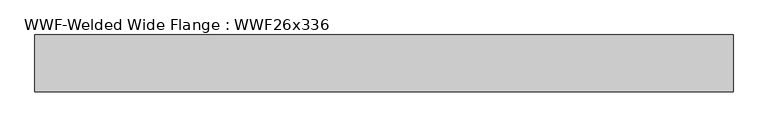
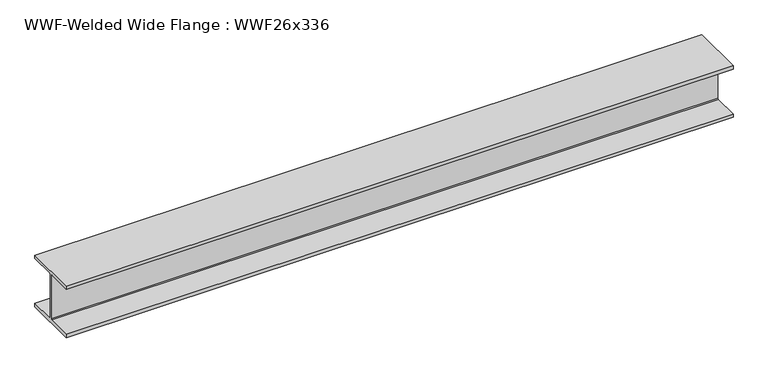
"""IFC4 building model written with IfcOpenShell, lengths in millimetres: beam geometry, WWF-Welded Wide Flange : WWF26x336."""

from ifc_helpers import new_model, si_unit, frame, origin, place, context, project, spatial, polyline, outline, extrude, source, transform, mapped, element, save


def wwf_welded_wide_flange_wwf26x336_1f70f701(model_context):
    return source(origin(), model_context, "Body", "SweptSolid", [
        extrude(outline(polyline([(324.993, -284.988), (324.993, -324.993), (-324.993, -324.993), (-324.993, -284.988), (-20.6375, -284.988), (-9.9949, -274.3454), (-9.9949, 274.3454), (-20.6375, 284.988), (-324.993, 284.988), (-324.993, 324.993), (324.993, 324.993), (324.993, 284.988), (20.6375, 284.988), (9.9949, 274.3454), (9.9949, -274.3454), (20.6375, -284.988), (324.993, -284.988)])), frame((-3934.8877112, 0.0, 0.0), z_axis=(1.0, 0.0, 0.0), x_axis=(0.0, 1.0, 0.0)), (0.0, 0.0, 1.0), 7999.1222788),
    ])


if __name__ == "__main__":
    model = new_model("IFC4")
    model_context = context("Model", 3, world=origin())
    ifc_project = project(units=[si_unit("LENGTHUNIT", "METRE", prefix="MILLI")], contexts=[model_context])
    site = spatial("IfcSite", under=ifc_project)
    building = spatial("IfcBuilding", under=site)
    placement = place(None, origin())
    wwf_welded_wide_flange_wwf26x336_shape = wwf_welded_wide_flange_wwf26x336_1f70f701(model_context)
    element("IfcBeam", 1, ObjectType="WWF-Welded Wide Flange : WWF26x336", at=placement, inside=building, context=model_context, shape_type="MappedRepresentation", body=[
        mapped(wwf_welded_wide_flange_wwf26x336_shape, transform((0.0, 0.0, 0.0), x_axis=(1.0, 0.0, 0.0), y_axis=(0.0, 1.0, 0.0), z_axis=(0.0, 0.0, 1.0))),
    ])
    save(model, "model.ifc")

# Revit data of these elements
# Type "WWF-Welded Wide Flange : WWF26x336"
#   Assembly Code = "B10"
#   Nominal d = "12"
#   W = 336
#   Length [instance default] = 1524 mm
#   bf = 649.986 mm
#   d = 649.986 mm
#   k = 20.638 mm
#   tf = 40.005 mm
#   tw = 19.99 mm
#   A = 0.0635483 m²
#   Structural Material [instance default] = Steel ASTM A572
# Element 1 (IfcBeam, "WWF-Welded Wide Flange : WWF26x336")
#   Structural Material = Metal - Steel 43-275
#   Materials on its faces: "Metal - Steel 43-275"
# Materials
#   "Steel ASTM A572": class "Metal", colour RGB 247 247 247, transparency 0, Description = "Structural steel, high strength low alloy, ASTM - A572 - 50", Cost = 0
#   "Metal - Steel 43-275": class "Metal", colour RGB 247 247 247, transparency 0, Cost = 0
